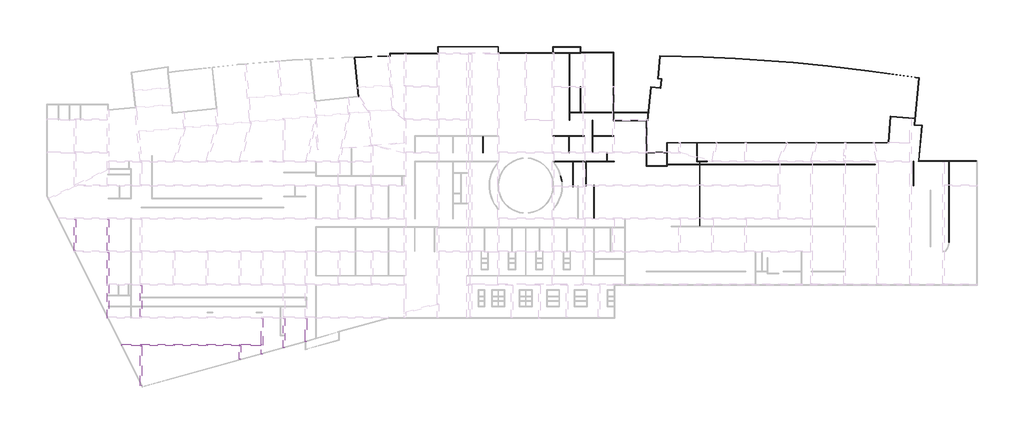
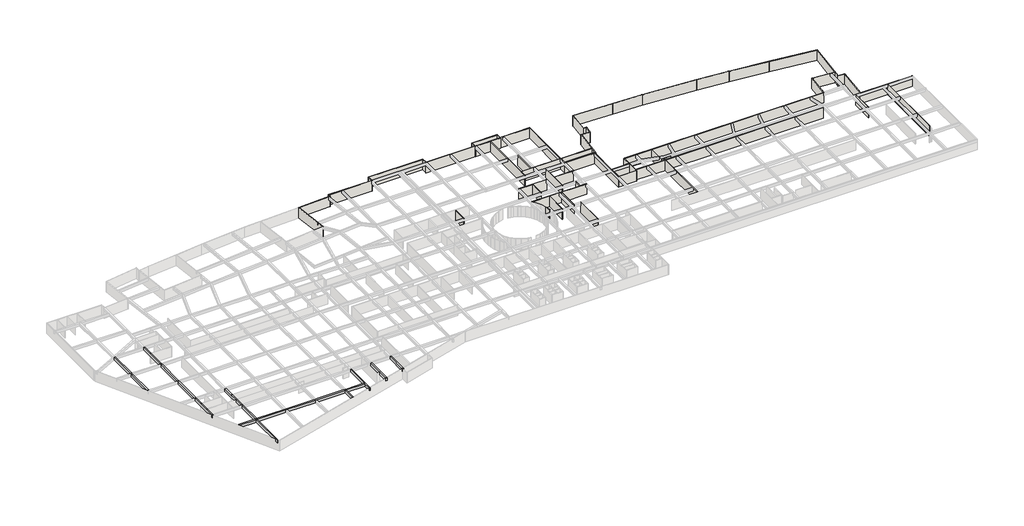
# One storey, part 4 of 8: 57 walls, 10 beams.
"""IFC4 building model written with IfcOpenShell, lengths in millimetres."""

from ifc_helpers import new_model, si_unit, frame, origin, origin_with_axes, place, context, project, spatial, polyline, outline, extrude, faceted_brep, element, save

model = new_model("IFC4")

# Units and contexts
model_context = context("Model", 3, world=origin())
ifc_project = project(units=[si_unit("LENGTHUNIT", "METRE", prefix="MILLI")], contexts=[model_context])

# Site, building, storey
site = spatial("IfcSite", under=ifc_project)
building = spatial("IfcBuilding", under=site)
storey = spatial("IfcBuildingStorey", under=building, Name="户型图", Elevation=0.0)

# Beams
placement = place(None, origin())
element("IfcBeam", 1, ObjectType="混凝土 - 矩形梁 : KL_beam", at=placement, inside=storey, context=model_context, shape_type="SweptSolid", body=[
    extrude(outline(polyline([(307553.8653555, -11261.3735096), (307153.8653555, -11261.3735096), (307153.8653555, -2661.3735096), (307553.8653555, -2661.3735096), (307553.8653555, -11261.3735096)])), frame((0.0, 0.0, 2500.0), z_axis=(0.0, 0.0, 1.0), x_axis=(1.0, 0.0, 0.0)), (0.0, 0.0, 1.0), 800.0),
    extrude(outline(polyline([(307153.8653555, 6215.0196927), (307401.078951, 6338.6264904), (307553.8653555, 6338.6264904), (307553.8653555, -2261.3735096), (307153.8653555, -2261.3735096), (307153.8653555, 6215.0196927)])), frame((0.0, 0.0, 2500.0), z_axis=(0.0, 0.0, 1.0), x_axis=(1.0, 0.0, 0.0)), (0.0, 0.0, 1.0), 800.0),
])
element("IfcBeam", 2, ObjectType="混凝土 - 矩形梁 : KL_beam", at=placement, inside=storey, context=model_context, shape_type="SweptSolid", body=[
    extrude(outline(polyline([(316153.8653576, 6338.6264904), (316553.8653576, 6338.6264904), (316553.8653576, -2261.3735096), (316153.8653576, -2261.3735096), (316153.8653576, 6338.6264904)])), frame((0.0, 0.0, 2500.0), z_axis=(0.0, 0.0, 1.0), x_axis=(1.0, 0.0, 0.0)), (0.0, 0.0, 1.0), 800.0),
    extrude(outline(polyline([(316553.8653576, -11261.3735096), (316153.8653576, -11261.3735096), (316153.8653576, -2661.3735096), (316553.8653576, -2661.3735096), (316553.8653576, -11261.3735096)])), frame((0.0, 0.0, 2500.0), z_axis=(0.0, 0.0, 1.0), x_axis=(1.0, 0.0, 0.0)), (0.0, 0.0, 1.0), 800.0),
])
element("IfcBeam", 3, ObjectType="混凝土 - 矩形梁 : KL_beam", at=placement, inside=storey, context=model_context, shape_type="Brep", body=[
    faceted_brep([(316153.8653576, -29635.5681734, 3300.0), (316553.8653576, -29635.5681734, 3300.0), (316553.8653576, -29235.5681734, 3300.0), (316553.8653576, -20661.3735124, 3300.0), (316553.8653576, -20261.3735124, 3300.0), (316553.8653576, -11661.3735096, 3300.0), (316153.8653576, -11661.3735096, 3300.0), (316153.8653576, -20261.3735124, 3300.0), (316153.8653576, -20661.3735124, 3300.0), (316153.8653576, -29635.5681734, 2500.0), (316153.8653576, -11661.3735096, 2500.0), (316153.8653576, -20261.3735124, 2500.0), (316153.8653576, -20661.3735124, 2500.0), (316553.8653576, -29635.5681734, 2500.0), (316553.8653576, -11661.3735096, 2500.0), (316553.8653576, -20261.3735124, 2500.0), (316553.8653576, -20661.3735124, 2500.0), (316553.8653576, -29235.5681734, 2500.0)], [[[0, 1, 2, 3, 4, 5, 6, 7, 8]], [[9, 0, 8, 7, 6, 10, 11, 12]], [[13, 9, 12, 11, 10, 14, 15, 16, 17]], [[1, 13, 17, 16, 15, 14, 5, 4, 3, 2]], [[6, 5, 14, 10]], [[1, 0, 9, 13]]]),
])
element("IfcBeam", 4, ObjectType="混凝土 - 矩形梁 : KL_beam", at=placement, inside=storey, context=model_context, shape_type="SweptSolid", body=[
    extrude(outline(polyline([(325153.8653576, -20661.3735124), (325553.8653576, -20661.3735124), (325553.8653576, -29235.5681734), (325153.8653576, -29235.5681734), (325153.8653576, -20661.3735124)])), frame((0.0, 0.0, 2500.0), z_axis=(0.0, 0.0, 1.0), x_axis=(1.0, 0.0, 0.0)), (0.0, 0.0, 1.0), 800.0),
    extrude(outline(polyline([(325153.8653576, -29635.5681734), (325553.8653576, -29635.5681734), (325553.8653576, -36750.8162358), (325153.8653576, -36750.8162358), (325153.8653576, -29635.5681734)])), frame((0.0, 0.0, 2500.0), z_axis=(0.0, 0.0, 1.0), x_axis=(1.0, 0.0, 0.0)), (0.0, 0.0, 1.0), 800.0),
])
element("IfcBeam", 5, ObjectType="混凝土 - 矩形梁 : KL_beam", at=placement, inside=storey, context=model_context, shape_type="SweptSolid", body=[
    extrude(outline(polyline([(325553.8653576, -48161.0948727), (325153.8653576, -48161.0948727), (325153.8653576, -37150.8162358), (325553.8653576, -37150.8162358), (325553.8653576, -48161.0948727)])), frame((0.0, 0.0, 2500.0), z_axis=(0.0, 0.0, 1.0), x_axis=(1.0, 0.0, 0.0)), (0.0, 0.0, 1.0), 800.0),
])
element("IfcBeam", 6, ObjectType="混凝土 - 矩形梁 : KL_beam", at=placement, inside=storey, context=model_context, shape_type="Brep", body=[
    faceted_brep([(320098.7260393, -36750.8162358, 3300.0), (320098.7260393, -36750.8162358, 2500.0), (320098.7260393, -37150.8162358, 2500.0), (320098.7260393, -37150.8162358, 3300.0), (325153.8653576, -37150.8162358, 3300.0), (325553.8653576, -37150.8162358, 3300.0), (334153.8653576, -37150.8162358, 3300.0), (334553.8653576, -37150.8162358, 3300.0), (343153.8653576, -37150.8162358, 3300.0), (343553.8653576, -37150.8162358, 3300.0), (352153.8653576, -37150.8162358, 3300.0), (352553.8653576, -37150.8162358, 3300.0), (358153.8653576, -37150.8162358, 3300.0), (358153.8653576, -36750.8162358, 3300.0), (352553.8653576, -36750.8162358, 3300.0), (352153.8653576, -36750.8162358, 3300.0), (343553.8653576, -36750.8162358, 3300.0), (343153.8653576, -36750.8162358, 3300.0), (334553.8653576, -36750.8162358, 3300.0), (334153.8653576, -36750.8162358, 3300.0), (325553.8653576, -36750.8162358, 3300.0), (325153.8653576, -36750.8162358, 3300.0), (325153.8653576, -37150.8162358, 2500.0), (325553.8653576, -37150.8162358, 2500.0), (334153.8653576, -37150.8162358, 2500.0), (334553.8653576, -37150.8162358, 2500.0), (343153.8653576, -37150.8162358, 2500.0), (343553.8653576, -37150.8162358, 2500.0), (352153.8653576, -37150.8162358, 2500.0), (352553.8653576, -37150.8162358, 2500.0), (358153.8653576, -37150.8162358, 2500.0), (325153.8653576, -36750.8162358, 2500.0), (325553.8653576, -36750.8162358, 2500.0), (334153.8653576, -36750.8162358, 2500.0), (334553.8653576, -36750.8162358, 2500.0), (343153.8653576, -36750.8162358, 2500.0), (343553.8653576, -36750.8162358, 2500.0), (352153.8653576, -36750.8162358, 2500.0), (352553.8653576, -36750.8162358, 2500.0), (358153.8653576, -36750.8162358, 2500.0)], [[[0, 1, 2, 3]], [[0, 3, 4, 5, 6, 7, 8, 9, 10, 11, 12, 13, 14, 15, 16, 17, 18, 19, 20, 21]], [[3, 2, 22, 23, 24, 25, 26, 27, 28, 29, 30, 12, 11, 10, 9, 8, 7, 6, 5, 4]], [[2, 1, 31, 32, 33, 34, 35, 36, 37, 38, 39, 30, 29, 28, 27, 26, 25, 24, 23, 22]], [[1, 0, 21, 20, 19, 18, 17, 16, 15, 14, 13, 39, 38, 37, 36, 35, 34, 33, 32, 31]], [[13, 12, 30, 39]]]),
])
element("IfcBeam", 7, ObjectType="混凝土 - 矩形梁 : KL_beam", at=placement, inside=storey, context=model_context, shape_type="SweptSolid", body=[
    extrude(outline(polyline([(352553.8653576, -40850.8162358), (352153.8653576, -40850.8162358), (352153.8653576, -37150.8162358), (352553.8653576, -37150.8162358), (352553.8653576, -40850.8162358)])), frame((0.0, 0.0, 2500.0), z_axis=(0.0, 0.0, 1.0), x_axis=(1.0, 0.0, 0.0)), (0.0, 0.0, 1.0), 800.0),
])
element("IfcBeam", 8, ObjectType="混凝土 - 矩形梁 : KL_beam", at=placement, inside=storey, context=model_context, shape_type="Brep", body=[
    faceted_brep([(358553.8653576, -39436.8004779, 3300.0), (358153.8653576, -39436.8004779, 3300.0), (358153.8653576, -39436.8004779, 2500.0), (358553.8653576, -39436.8004779, 2500.0), (358553.8653576, -29635.5681734, 3300.0), (358153.8653576, -29635.5681734, 3300.0), (358153.8653576, -36750.8162358, 3300.0), (358153.8653576, -37150.8162358, 3300.0), (358153.8653576, -29635.5681734, 2500.0), (358153.8653576, -36750.8162358, 2500.0), (358153.8653576, -37150.8162358, 2500.0), (358553.8653576, -29635.5681734, 2500.0)], [[[0, 1, 2, 3]], [[1, 0, 4, 5, 6, 7]], [[2, 1, 7, 6, 5, 8, 9, 10]], [[3, 2, 10, 9, 8, 11]], [[0, 3, 11, 4]], [[5, 4, 11, 8]]]),
])
element("IfcBeam", 9, ObjectType="混凝土 - 矩形梁 : KL_beam", at=placement, inside=storey, context=model_context, shape_type="SweptSolid", body=[
    extrude(outline(polyline([(364553.8653576, -37769.9671448), (364153.8653576, -37769.9671448), (364153.8653576, -29635.5681734), (364553.8653576, -29635.5681734), (364553.8653576, -37769.9671448)])), frame((0.0, 0.0, 2500.0), z_axis=(0.0, 0.0, 1.0), x_axis=(1.0, 0.0, 0.0)), (0.0, 0.0, 1.0), 800.0),
])
element("IfcBeam", 10, ObjectType="混凝土 - 矩形梁 : KL_beam", at=placement, inside=storey, context=model_context, shape_type="SweptSolid", body=[
    extrude(outline(polyline([(370553.8653576, -36103.6338116), (370153.8653576, -36103.6338116), (370153.8653576, -29635.5681734), (370553.8653576, -29635.5681734), (370553.8653576, -36103.6338116)])), frame((0.0, 0.0, 2500.0), z_axis=(0.0, 0.0, 1.0), x_axis=(1.0, 0.0, 0.0)), (0.0, 0.0, 1.0), 800.0),
])

# Walls
element("IfcWall", 11, ObjectType="所有墙体", at=placement, inside=storey, context=model_context, shape_type="Brep", body=[
    faceted_brep([(553458.7450641, 13292.21774, 0.0), (537684.2235741, 13292.21774, 0.0), (537563.7651936, 13292.21774, 0.0), (537563.7651936, 13292.21774, 3300.0), (537684.2235741, 13292.21774, 3300.0), (553458.7450641, 13292.21774, 3300.0), (553458.7450641, 13172.21774, 0.0), (553458.7450641, 13172.21774, 3300.0), (537553.266554, 13172.21774, 3300.0), (537553.266554, 13172.21774, 0.0)], [[[0, 1, 2, 3, 4, 5]], [[6, 7, 8, 9]], [[2, 1, 0, 6, 9]], [[5, 4, 3, 8, 7]], [[0, 5, 7, 6]], [[3, 2, 9, 8]]]),
])
element("IfcWall", 12, ObjectType="所有墙体", at=placement, inside=storey, context=model_context, shape_type="Brep", body=[
    faceted_brep([(537684.2235741, 13292.21774, 0.0), (538529.2876848, 22951.3447265, 0.0), (538529.2876848, 22951.3447265, 3300.0), (537684.2235741, 13292.21774, 3300.0), (537563.7651936, 13292.21774, 0.0), (537563.7651936, 13292.21774, 3300.0), (538399.3397888, 22842.8790687, 3300.0), (538409.7986189, 22962.4240435, 3300.0), (538409.7986189, 22962.4240435, 0.0), (538399.3397888, 22842.8790687, 0.0)], [[[0, 1, 2, 3]], [[4, 5, 6, 7, 8, 9]], [[1, 0, 4, 9, 8]], [[3, 2, 7, 6, 5]], [[0, 3, 5, 4]], [[2, 1, 8, 7]]]),
])
element("IfcWall", 13, ObjectType="所有墙体", at=placement, inside=storey, context=model_context, shape_type="Brep", body=[
    faceted_brep([(538409.7986189, 22962.4240435, 0.0), (536538.1394552, 23135.9688357, 0.0), (536418.6519996, 23147.0480034, 0.0), (536418.6519996, 23147.0480034, 3300.0), (536538.1394552, 23135.9688357, 3300.0), (538409.7986189, 22962.4240435, 3300.0), (538399.3397888, 22842.8790687, 0.0), (538399.3397888, 22842.8790687, 3300.0), (536407.572832, 23027.5605478, 3300.0), (536407.572832, 23027.5605478, 0.0)], [[[0, 1, 2, 3, 4, 5]], [[6, 7, 8, 9]], [[2, 1, 0, 6, 9]], [[5, 4, 3, 8, 7]], [[0, 5, 7, 6]], [[3, 2, 9, 8]]]),
])
element("IfcWall", 14, ObjectType="所有墙体", at=placement, inside=storey, context=model_context, shape_type="Brep", body=[
    faceted_brep([(536538.1394552, 23135.9688357, 0.0), (537732.2315967, 36014.1051945, 0.0), (537732.2315967, 36014.1051945, 3300.0), (536538.1394552, 23135.9688357, 3300.0), (536418.6519996, 23147.0480034, 0.0), (536418.6519996, 23147.0480034, 3300.0), (536566.2044403, 24738.382864, 3300.0), (536577.283608, 24857.8703196, 3300.0), (537602.1010394, 35910.3998237, 3300.0), (537613.1891402, 36029.9836226, 3300.0), (537613.1891402, 36029.9836226, 0.0), (537602.1010394, 35910.3998237, 0.0), (536577.283608, 24857.8703196, 0.0), (536566.2044403, 24738.382864, 0.0)], [[[0, 1, 2, 3]], [[4, 5, 6, 7, 8, 9, 10, 11, 12, 13]], [[1, 0, 4, 13, 12, 11, 10]], [[3, 2, 9, 8, 7, 6, 5]], [[0, 3, 5, 4]], [[2, 1, 10, 9]]]),
])
element("IfcWall", 15, ObjectType="所有墙体", at=placement, inside=storey, context=model_context, shape_type="SweptSolid", body=[
    extrude(outline(polyline([(524037.26481, 37840.8025861), (537613.1891402, 36029.9836226), (537602.1010394, 35910.3998237), (524021.9834406, 37721.7781046), (524037.26481, 37840.8025861)])), origin_with_axes(), (0.0, 0.0, 1.0), 3300.0),
])
element("IfcWall", 16, ObjectType="所有墙体", at=placement, inside=storey, context=model_context, shape_type="SweptSolid", body=[
    extrude(outline(polyline([(512770.3311829, 39231.1267428), (524037.26481, 37840.8025861), (524021.9834406, 37721.7781046), (512757.0555613, 39111.8547548), (512770.3311829, 39231.1267428)])), origin_with_axes(), (0.0, 0.0, 1.0), 3300.0),
])
element("IfcWall", 17, ObjectType="所有墙体", at=placement, inside=storey, context=model_context, shape_type="SweptSolid", body=[
    extrude(outline(polyline([(503394.9424706, 40161.5809347), (512770.3311829, 39231.1267428), (512757.0555613, 39111.8547548), (503384.5461664, 40042.0231907), (503394.9424706, 40161.5809347)])), origin_with_axes(), (0.0, 0.0, 1.0), 3300.0),
])
element("IfcWall", 18, ObjectType="所有墙体", at=placement, inside=storey, context=model_context, shape_type="SweptSolid", body=[
    extrude(outline(polyline([(487600.1090231, 41341.3659197), (503394.9424706, 40161.5809347), (503384.5461664, 40042.0231907), (487593.4285844, 41221.5306216), (487600.1090231, 41341.3659197)])), origin_with_axes(), (0.0, 0.0, 1.0), 3300.0),
])
element("IfcWall", 19, ObjectType="所有墙体", at=placement, inside=storey, context=model_context, shape_type="SweptSolid", body=[
    extrude(outline(polyline([(478777.792417, 41666.3723956), (487600.1090231, 41341.3659197), (487593.4285844, 41221.5306216), (478774.1034736, 41546.4268934), (478777.792417, 41666.3723956)])), origin_with_axes(), (0.0, 0.0, 1.0), 3300.0),
])
element("IfcWall", 20, ObjectType="所有墙体", at=placement, inside=storey, context=model_context, shape_type="Brep", body=[
    faceted_brep([(478777.792417, 41666.3723956, 0.0), (466951.5716276, 41958.1662767, 0.0), (466951.5716276, 41958.1662767, 3300.0), (478777.792417, 41666.3723956, 3300.0), (478774.1034736, 41546.4268934, 0.0), (478774.1034736, 41546.4268934, 3300.0), (467061.2925699, 41835.4225593, 3300.0), (466941.0937395, 41838.3882813, 3300.0), (466941.0937395, 41838.3882813, 0.0), (467061.2925699, 41835.4225593, 0.0)], [[[0, 1, 2, 3]], [[4, 5, 6, 7, 8, 9]], [[1, 0, 4, 9, 8]], [[3, 2, 7, 6, 5]], [[0, 3, 5, 4]], [[2, 1, 8, 7]]]),
])
element("IfcWall", 21, ObjectType="所有墙体", at=placement, inside=storey, context=model_context, shape_type="Brep", body=[
    faceted_brep([(466941.0937395, 41838.3882813, 0.0), (466401.1341207, 35665.8389465, 0.0), (466401.1341207, 35665.8389465, 3300.0), (466941.0937395, 41838.3882813, 3300.0), (467061.2925699, 41835.4225593, 0.0), (467061.2925699, 41835.4225593, 3300.0), (466531.1348575, 35774.9237362, 3300.0), (466520.6774844, 35655.3802573, 3300.0), (466520.6774844, 35655.3802573, 0.0), (466531.1348575, 35774.9237362, 0.0)], [[[0, 1, 2, 3]], [[4, 5, 6, 7, 8, 9]], [[1, 0, 4, 9, 8]], [[3, 2, 7, 6, 5]], [[0, 3, 5, 4]], [[2, 1, 8, 7]]]),
])
element("IfcWall", 22, ObjectType="所有墙体", at=placement, inside=storey, context=model_context, shape_type="Brep", body=[
    faceted_brep([(466520.6774844, 35655.3802573, 0.0), (467298.2016586, 35587.3557065, 0.0), (467417.7450224, 35576.8970174, 0.0), (467417.7450224, 35576.8970174, 3300.0), (467298.2016586, 35587.3557065, 3300.0), (466520.6774844, 35655.3802573, 3300.0), (466531.1348575, 35774.9237362, 0.0), (466531.1348575, 35774.9237362, 3300.0), (467428.2037115, 35696.4403811, 3300.0), (467428.2037115, 35696.4403811, 0.0)], [[[0, 1, 2, 3, 4, 5]], [[6, 7, 8, 9]], [[2, 1, 0, 6, 9]], [[5, 4, 3, 8, 7]], [[0, 5, 7, 6]], [[3, 2, 9, 8]]]),
])
element("IfcWall", 23, ObjectType="所有墙体", at=placement, inside=storey, context=model_context, shape_type="Brep", body=[
    faceted_brep([(467298.2016586, 35587.3557065, 0.0), (467095.1766515, 33266.769256, 0.0), (467084.7179624, 33147.2258923, 0.0), (467084.7179624, 33147.2258923, 3300.0), (467095.1766515, 33266.769256, 3300.0), (467298.2016586, 35587.3557065, 3300.0), (467417.7450224, 35576.8970174, 0.0), (467417.7450224, 35576.8970174, 3300.0), (467204.2613261, 33136.7672031, 3300.0), (467204.2613261, 33136.7672031, 0.0)], [[[0, 1, 2, 3, 4, 5]], [[6, 7, 8, 9]], [[2, 1, 0, 6, 9]], [[5, 4, 3, 8, 7]], [[0, 5, 7, 6]], [[3, 2, 9, 8]]]),
])
element("IfcWall", 24, ObjectType="所有墙体", at=placement, inside=storey, context=model_context, shape_type="Brep", body=[
    faceted_brep([(467095.1766515, 33266.769256, 0.0), (464505.7177262, 33493.3175566, 0.0), (464505.7177262, 33493.3175566, 3300.0), (467095.1766515, 33266.769256, 3300.0), (467084.7179624, 33147.2258923, 0.0), (467084.7179624, 33147.2258923, 3300.0), (464613.5078213, 33363.4287647, 3300.0), (464493.9573711, 33373.8880738, 3300.0), (464493.9573711, 33373.8880738, 0.0), (464613.5078213, 33363.4287647, 0.0)], [[[0, 1, 2, 3]], [[4, 5, 6, 7, 8, 9]], [[1, 0, 4, 9, 8]], [[3, 2, 7, 6, 5]], [[0, 3, 5, 4]], [[2, 1, 8, 7]]]),
])
element("IfcWall", 25, ObjectType="所有墙体", at=placement, inside=storey, context=model_context, shape_type="Brep", body=[
    faceted_brep([(464493.9573711, 33373.8880738, 0.0), (463826.7897593, 26598.6264677, 0.0), (463814.9732246, 26478.6264677, 0.0), (463600.3061777, 24298.6264562, 0.0), (463588.489643, 24178.6264562, 0.0), (463588.489643, 24178.6264562, 3300.0), (463600.3061777, 24298.6264562, 3300.0), (463814.9732246, 26478.6264677, 3300.0), (463826.7897593, 26598.6264677, 3300.0), (464493.9573711, 33373.8880738, 3300.0), (464613.5078213, 33363.4287647, 0.0), (464613.5078213, 33363.4287647, 3300.0), (463709.0700332, 24178.6264562, 3300.0), (463709.0700332, 24178.6264562, 0.0)], [[[0, 1, 2, 3, 4, 5, 6, 7, 8, 9]], [[10, 11, 12, 13]], [[4, 3, 2, 1, 0, 10, 13]], [[9, 8, 7, 6, 5, 12, 11]], [[0, 9, 11, 10]], [[5, 4, 13, 12]]]),
])
element("IfcWall", 26, ObjectType="所有墙体", at=placement, inside=storey, context=model_context, shape_type="Brep", body=[
    faceted_brep([(463600.3061777, 24298.6264562, 0.0), (454413.8653571, 24298.6264562, 0.0), (454293.8653571, 24298.6264562, 0.0), (454293.8653571, 24298.6264562, 3300.0), (454413.8653571, 24298.6264562, 3300.0), (463600.3061777, 24298.6264562, 3300.0), (463588.489643, 24178.6264562, 0.0), (463588.489643, 24178.6264562, 3300.0), (463413.8653576, 24178.6264562, 3300.0), (463293.8653576, 24178.6264562, 3300.0), (454293.8653571, 24178.6264562, 3300.0), (454293.8653571, 24178.6264562, 0.0), (463293.8653576, 24178.6264562, 0.0), (463413.8653576, 24178.6264562, 0.0)], [[[0, 1, 2, 3, 4, 5]], [[6, 7, 8, 9, 10, 11, 12, 13]], [[2, 1, 0, 6, 13, 12, 11]], [[5, 4, 3, 10, 9, 8, 7]], [[0, 5, 7, 6]], [[3, 2, 11, 10]]]),
])
element("IfcWall", 27, ObjectType="所有墙体", at=placement, inside=storey, context=model_context, shape_type="Brep", body=[
    faceted_brep([(454413.8653571, 24298.6264562, 0.0), (454413.8653571, 26478.6264677, 0.0), (454413.8653571, 26598.6264677, 0.0), (454413.8653571, 42898.6264606, 0.0), (454413.8653571, 42898.6264606, 3300.0), (454413.8653571, 26598.6264677, 3300.0), (454413.8653571, 26478.6264677, 3300.0), (454413.8653571, 24298.6264562, 3300.0), (454293.8653571, 24298.6264562, 0.0), (454293.8653571, 24298.6264562, 3300.0), (454293.8653571, 26478.6264677, 3300.0), (454293.8653571, 26598.6264677, 3300.0), (454293.8653571, 42778.6264606, 3300.0), (454293.8653571, 42898.6264606, 3300.0), (454293.8653571, 42898.6264606, 0.0), (454293.8653571, 42778.6264606, 0.0), (454293.8653571, 26598.6264677, 0.0), (454293.8653571, 26478.6264677, 0.0)], [[[0, 1, 2, 3, 4, 5, 6, 7]], [[8, 9, 10, 11, 12, 13, 14, 15, 16, 17]], [[3, 2, 1, 0, 8, 17, 16, 15, 14]], [[7, 6, 5, 4, 13, 12, 11, 10, 9]], [[0, 7, 9, 8]], [[4, 3, 14, 13]]]),
])
element("IfcWall", 28, ObjectType="所有墙体", at=placement, inside=storey, context=model_context, shape_type="Brep", body=[
    faceted_brep([(454293.8653571, 42898.6264606, 0.0), (445413.8653571, 42898.6264606, 0.0), (445293.8653571, 42898.6264606, 0.0), (445293.8653571, 42898.6264606, 3300.0), (445413.8653571, 42898.6264606, 3300.0), (454293.8653571, 42898.6264606, 3300.0), (454293.8653571, 42778.6264606, 0.0), (454293.8653571, 42778.6264606, 3300.0), (445293.8653571, 42778.6264606, 3300.0), (445293.8653571, 42778.6264606, 0.0)], [[[0, 1, 2, 3, 4, 5]], [[6, 7, 8, 9]], [[2, 1, 0, 6, 9]], [[5, 4, 3, 8, 7]], [[0, 5, 7, 6]], [[3, 2, 9, 8]]]),
])
element("IfcWall", 29, ObjectType="所有墙体", at=placement, inside=storey, context=model_context, shape_type="Brep", body=[
    faceted_brep([(445413.8653571, 42898.6264606, 0.0), (445413.8653571, 44395.5707464, 0.0), (445413.8653571, 44395.5707464, 3300.0), (445413.8653571, 42898.6264606, 3300.0), (445293.8653571, 42898.6264606, 0.0), (445293.8653571, 42898.6264606, 3300.0), (445293.8653571, 44275.5707464, 3300.0), (445293.8653571, 44395.5707464, 3300.0), (445293.8653571, 44395.5707464, 0.0), (445293.8653571, 44275.5707464, 0.0)], [[[0, 1, 2, 3]], [[4, 5, 6, 7, 8, 9]], [[1, 0, 4, 9, 8]], [[3, 2, 7, 6, 5]], [[0, 3, 5, 4]], [[2, 1, 8, 7]]]),
])
element("IfcWall", 30, ObjectType="所有墙体", at=placement, inside=storey, context=model_context, shape_type="Brep", body=[
    faceted_brep([(445293.8653571, 44395.5707464, 0.0), (437693.8653571, 44395.5707464, 0.0), (437693.8653571, 44395.5707464, 3300.0), (445293.8653571, 44395.5707464, 3300.0), (445293.8653571, 44275.5707464, 0.0), (445293.8653571, 44275.5707464, 3300.0), (437813.8653571, 44275.5707464, 3300.0), (437693.8653571, 44275.5707464, 3300.0), (437693.8653571, 44275.5707464, 0.0), (437813.8653571, 44275.5707464, 0.0)], [[[0, 1, 2, 3]], [[4, 5, 6, 7, 8, 9]], [[1, 0, 4, 9, 8]], [[3, 2, 7, 6, 5]], [[0, 3, 5, 4]], [[2, 1, 8, 7]]]),
])
element("IfcWall", 31, ObjectType="所有墙体", at=placement, inside=storey, context=model_context, shape_type="Brep", body=[
    faceted_brep([(437693.8653571, 44275.5707464, 0.0), (437693.8653571, 42795.5707464, 0.0), (437693.8653571, 42675.5707464, 0.0), (437693.8653571, 42675.5707464, 3300.0), (437693.8653571, 42795.5707464, 3300.0), (437693.8653571, 44275.5707464, 3300.0), (437813.8653571, 44275.5707464, 0.0), (437813.8653571, 44275.5707464, 3300.0), (437813.8653571, 42735.5707464, 3300.0), (437813.8653571, 42675.5707464, 3300.0), (437813.8653571, 42675.5707464, 0.0), (437813.8653571, 42735.5707464, 0.0)], [[[0, 1, 2, 3, 4, 5]], [[6, 7, 8, 9, 10, 11]], [[2, 1, 0, 6, 11, 10]], [[5, 4, 3, 9, 8, 7]], [[0, 5, 7, 6]], [[3, 2, 10, 9]]]),
])
element("IfcWall", 32, ObjectType="所有墙体", at=placement, inside=storey, context=model_context, shape_type="Brep", body=[
    faceted_brep([(437693.8653571, 42795.5707464, 0.0), (422913.8653571, 42795.5707464, 0.0), (422793.8653571, 42795.5707464, 0.0), (422793.8653571, 42795.5707464, 3300.0), (422913.8653571, 42795.5707464, 3300.0), (437693.8653571, 42795.5707464, 3300.0), (437693.8653571, 42675.5707464, 0.0), (437693.8653571, 42675.5707464, 3300.0), (422793.8653571, 42675.5707464, 3300.0), (422793.8653571, 42675.5707464, 0.0)], [[[0, 1, 2, 3, 4, 5]], [[6, 7, 8, 9]], [[2, 1, 0, 6, 9]], [[5, 4, 3, 8, 7]], [[0, 5, 7, 6]], [[3, 2, 9, 8]]]),
])
element("IfcWall", 33, ObjectType="所有墙体", at=placement, inside=storey, context=model_context, shape_type="Brep", body=[
    faceted_brep([(422913.8653571, 42795.5707464, 0.0), (422913.8653571, 44495.5707464, 0.0), (422913.8653571, 44495.5707464, 3300.0), (422913.8653571, 42795.5707464, 3300.0), (422793.8653571, 42795.5707464, 0.0), (422793.8653571, 42795.5707464, 3300.0), (422793.8653571, 44375.5707464, 3300.0), (422793.8653571, 44495.5707464, 3300.0), (422793.8653571, 44495.5707464, 0.0), (422793.8653571, 44375.5707464, 0.0)], [[[0, 1, 2, 3]], [[4, 5, 6, 7, 8, 9]], [[1, 0, 4, 9, 8]], [[3, 2, 7, 6, 5]], [[0, 3, 5, 4]], [[2, 1, 8, 7]]]),
])
element("IfcWall", 34, ObjectType="所有墙体", at=placement, inside=storey, context=model_context, shape_type="Brep", body=[
    faceted_brep([(422793.8653571, 44495.5707464, 0.0), (406293.8653571, 44495.5707464, 0.0), (406293.8653571, 44495.5707464, 3300.0), (422793.8653571, 44495.5707464, 3300.0), (422793.8653571, 44375.5707464, 0.0), (422793.8653571, 44375.5707464, 3300.0), (406413.8653571, 44375.5707464, 3300.0), (406293.8653571, 44375.5707464, 3300.0), (406293.8653571, 44375.5707464, 0.0), (406413.8653571, 44375.5707464, 0.0)], [[[0, 1, 2, 3]], [[4, 5, 6, 7, 8, 9]], [[1, 0, 4, 9, 8]], [[3, 2, 7, 6, 5]], [[0, 3, 5, 4]], [[2, 1, 8, 7]]]),
])
element("IfcWall", 35, ObjectType="所有墙体", at=placement, inside=storey, context=model_context, shape_type="Brep", body=[
    faceted_brep([(406293.8653571, 44375.5707464, 0.0), (406293.8653571, 42695.5707464, 0.0), (406293.8653571, 42575.5707464, 0.0), (406293.8653571, 42575.5707464, 3300.0), (406293.8653571, 42695.5707464, 3300.0), (406293.8653571, 44375.5707464, 3300.0), (406413.8653571, 44375.5707464, 0.0), (406413.8653571, 44375.5707464, 3300.0), (406413.8653571, 42575.5707464, 3300.0), (406413.8653571, 42575.5707464, 0.0)], [[[0, 1, 2, 3, 4, 5]], [[6, 7, 8, 9]], [[2, 1, 0, 6, 9]], [[5, 4, 3, 8, 7]], [[0, 5, 7, 6]], [[3, 2, 9, 8]]]),
])
element("IfcWall", 36, ObjectType="所有墙体", at=placement, inside=storey, context=model_context, shape_type="Brep", body=[
    faceted_brep([(406293.8653571, 42695.5707464, 0.0), (393193.8653571, 42695.5707464, 0.0), (393193.8653571, 42695.5707464, 3300.0), (406293.8653571, 42695.5707464, 3300.0), (406293.8653571, 42575.5707464, 0.0), (406293.8653571, 42575.5707464, 3300.0), (393313.8653571, 42575.5707464, 3300.0), (393193.8653571, 42575.5707464, 3300.0), (393193.8653571, 42575.5707464, 0.0), (393313.8653571, 42575.5707464, 0.0)], [[[0, 1, 2, 3]], [[4, 5, 6, 7, 8, 9]], [[1, 0, 4, 9, 8]], [[3, 2, 7, 6, 5]], [[0, 3, 5, 4]], [[2, 1, 8, 7]]]),
])
element("IfcWall", 37, ObjectType="所有墙体", at=placement, inside=storey, context=model_context, shape_type="Brep", body=[
    faceted_brep([(393193.8653571, 42575.5707464, 0.0), (393193.8653571, 41993.3912245, 0.0), (393193.8653571, 41873.3090682, 0.0), (393193.8653571, 41873.3090682, 3300.0), (393193.8653571, 41993.3912245, 3300.0), (393193.8653571, 42575.5707464, 3300.0), (393313.8653571, 42575.5707464, 0.0), (393313.8653571, 42575.5707464, 3300.0), (393313.8653571, 41877.7502684, 3300.0), (393313.8653571, 41877.7502684, 0.0)], [[[0, 1, 2, 3, 4, 5]], [[6, 7, 8, 9]], [[2, 1, 0, 6, 9]], [[5, 4, 3, 8, 7]], [[0, 5, 7, 6]], [[3, 2, 9, 8]]]),
])
element("IfcWall", 38, ObjectType="所有墙体", at=placement, inside=storey, context=model_context, shape_type="Brep", body=[
    faceted_brep([(393193.8653571, 41993.3912245, 0.0), (383558.0584634, 41636.7699948, 0.0), (383558.0584634, 41636.7699948, 3300.0), (393193.8653571, 41993.3912245, 3300.0), (393193.8653571, 41873.3090682, 0.0), (393193.8653571, 41873.3090682, 3300.0), (383626.8769002, 41519.2348089, 3300.0), (383562.9450973, 41516.8686928, 3300.0), (383562.9450973, 41516.8686928, 0.0), (383626.8769002, 41519.2348089, 0.0)], [[[0, 1, 2, 3]], [[4, 5, 6, 7, 8, 9]], [[1, 0, 4, 9, 8]], [[3, 2, 7, 6, 5]], [[0, 3, 5, 4]], [[2, 1, 8, 7]]]),
])
element("IfcWall", 39, ObjectType="所有墙体", at=placement, inside=storey, context=model_context, shape_type="Brep", body=[
    faceted_brep([(384756.3754813, 30760.3408142, 0.0), (383626.8769002, 41519.2348089, 0.0), (383626.8769002, 41519.2348089, 3300.0), (384756.3754813, 30760.3408142, 3300.0), (384637.0313479, 30747.8117356, 0.0), (384637.0313479, 30747.8117356, 3300.0), (384624.5022692, 30867.155869, 3300.0), (383506.7284721, 41514.3669361, 3300.0), (383506.7284721, 41514.3669361, 0.0), (384624.5022692, 30867.155869, 0.0), (383562.9450973, 41516.8686928, 0.0), (383562.9450972, 41516.8686928, 3300.0)], [[[0, 1, 2, 3]], [[4, 5, 6, 7, 8, 9]], [[1, 0, 4, 9, 8, 10]], [[3, 2, 11, 7, 6, 5]], [[2, 1, 10, 11]], [[10, 8, 7, 11]], [[0, 3, 5, 4]]]),
])
element("IfcWall", 40, ObjectType="所有墙体", at=placement, inside=storey, context=model_context, shape_type="Brep", body=[
    faceted_brep([(463293.8653576, 24178.6264562, 0.0), (463293.8653576, 11778.6265283, 0.0), (463293.8653576, 11778.6265283, 3300.0), (463293.8653576, 24178.6264562, 3300.0), (463413.8653576, 24178.6264562, 0.0), (463413.8653576, 24178.6264562, 3300.0), (463413.8653576, 15598.6264904, 3300.0), (463413.8653576, 15478.6264904, 3300.0), (463413.8653576, 11898.6265283, 3300.0), (463413.8653576, 11778.6265283, 3300.0), (463413.8653576, 11778.6265283, 0.0), (463413.8653576, 11898.6265283, 0.0), (463413.8653576, 15478.6264904, 0.0), (463413.8653576, 15598.6264904, 0.0)], [[[0, 1, 2, 3]], [[4, 5, 6, 7, 8, 9, 10, 11, 12, 13]], [[1, 0, 4, 13, 12, 11, 10]], [[3, 2, 9, 8, 7, 6, 5]], [[0, 3, 5, 4]], [[2, 1, 10, 9]]]),
])
element("IfcWall", 41, ObjectType="所有墙体", at=placement, inside=storey, context=model_context, shape_type="SweptSolid", body=[
    extrude(outline(polyline([(468793.8653361, 15478.6264904), (463413.8653576, 15478.6264904), (463413.8653576, 15598.6264904), (468793.8653361, 15598.6264904), (468793.8653361, 15478.6264904)])), origin_with_axes(), (0.0, 0.0, 1.0), 3300.0),
])
element("IfcWall", 42, ObjectType="所有墙体", at=placement, inside=storey, context=model_context, shape_type="Brep", body=[
    faceted_brep([(468913.8653361, 11778.6265283, 0.0), (468913.8653361, 18178.6264904, 0.0), (468913.8653361, 18298.6264904, 0.0), (468913.8653361, 18298.6264904, 3300.0), (468913.8653361, 18178.6264904, 3300.0), (468913.8653361, 11778.6265283, 3300.0), (468793.8653361, 11778.6265283, 0.0), (468793.8653361, 11778.6265283, 3300.0), (468793.8653361, 11898.6265283, 3300.0), (468793.8653361, 15478.6264904, 3300.0), (468793.8653361, 15598.6264904, 3300.0), (468793.8653361, 18298.6264904, 3300.0), (468793.8653361, 18298.6264904, 0.0), (468793.8653361, 15598.6264904, 0.0), (468793.8653361, 15478.6264904, 0.0), (468793.8653361, 11898.6265283, 0.0)], [[[0, 1, 2, 3, 4, 5]], [[6, 7, 8, 9, 10, 11, 12, 13, 14, 15]], [[2, 1, 0, 6, 15, 14, 13, 12]], [[5, 4, 3, 11, 10, 9, 8, 7]], [[3, 2, 12, 11]], [[0, 5, 7, 6]]]),
])
element("IfcWall", 43, ObjectType="所有墙体", at=placement, inside=storey, context=model_context, shape_type="Brep", body=[
    faceted_brep([(468913.8653361, 18178.6264904, 0.0), (477093.8653576, 18178.6264904, 0.0), (477213.8653576, 18178.6264904, 0.0), (529386.6252053, 18178.6264904, 0.0), (529386.6252053, 18178.6264904, 3300.0), (477213.8653576, 18178.6264904, 3300.0), (477093.8653576, 18178.6264904, 3300.0), (468913.8653361, 18178.6264904, 3300.0), (468913.8653361, 18298.6264904, 0.0), (468913.8653361, 18298.6264904, 3300.0), (529276.7559158, 18298.6264904, 3300.0), (529397.2229767, 18298.6264904, 3300.0), (529397.2229767, 18298.6264904, 0.0), (529276.7559158, 18298.6264904, 0.0)], [[[0, 1, 2, 3, 4, 5, 6, 7]], [[8, 9, 10, 11, 12, 13]], [[3, 2, 1, 0, 8, 13, 12]], [[7, 6, 5, 4, 11, 10, 9]], [[0, 7, 9, 8]], [[4, 3, 12, 11]]]),
])
element("IfcWall", 44, ObjectType="所有墙体", at=placement, inside=storey, context=model_context, shape_type="Brep", body=[
    faceted_brep([(529397.2229767, 18298.6264904, 0.0), (530019.5574453, 25345.4039043, 0.0), (530030.1142291, 25464.9397966, 0.0), (530030.1142291, 25464.9397966, 3300.0), (530019.5574453, 25345.4039043, 3300.0), (529397.2229767, 18298.6264904, 3300.0), (529276.7559158, 18298.6264904, 0.0), (529276.7559158, 18298.6264904, 3300.0), (529910.6256316, 25476.0190701, 3300.0), (529910.6256316, 25476.0190701, 0.0)], [[[0, 1, 2, 3, 4, 5]], [[6, 7, 8, 9]], [[2, 1, 0, 6, 9]], [[5, 4, 3, 8, 7]], [[0, 5, 7, 6]], [[3, 2, 9, 8]]]),
])
element("IfcWall", 45, ObjectType="所有墙体", at=placement, inside=storey, context=model_context, shape_type="SweptSolid", body=[
    extrude(outline(polyline([(536566.2044403, 24738.382864), (530019.5574453, 25345.4039043), (530030.1142291, 25464.9397966), (536577.283608, 24857.8703196), (536566.2044403, 24738.382864)])), origin_with_axes(), (0.0, 0.0, 1.0), 3300.0),
])
element("IfcWall", 46, ObjectType="所有墙体", at=placement, inside=storey, context=model_context, shape_type="SweptSolid", body=[
    extrude(outline(polyline([(463413.8653576, 11898.6265283), (468793.8653361, 11898.6265283), (468793.8653361, 11778.6265283), (463413.8653576, 11778.6265283), (463413.8653576, 11898.6265283)])), origin_with_axes(), (0.0, 0.0, 1.0), 3300.0),
])
element("IfcWall", 47, ObjectType="所有墙体", at=placement, inside=storey, context=model_context, shape_type="Brep", body=[
    faceted_brep([(469204.0947142, 12228.624256, 0.0), (477798.5776142, 12228.624256, 0.0), (477918.5776142, 12228.624256, 0.0), (525704.0947142, 12228.624256, 0.0), (525704.0947142, 12228.624256, 3300.0), (477918.5776142, 12228.624256, 3300.0), (477798.5776142, 12228.624256, 3300.0), (469204.0947142, 12228.624256, 3300.0), (469204.0947142, 12348.624256, 0.0), (469204.0947142, 12348.624256, 3300.0), (477798.5776142, 12348.624256, 3300.0), (477918.5776142, 12348.624256, 3300.0), (525704.0947142, 12348.624256, 3300.0), (525704.0947142, 12348.624256, 0.0), (477918.5776142, 12348.624256, 0.0), (477798.5776142, 12348.624256, 0.0)], [[[0, 1, 2, 3, 4, 5, 6, 7]], [[8, 9, 10, 11, 12, 13, 14, 15]], [[3, 2, 1, 0, 8, 15, 14, 13]], [[4, 3, 13, 12]], [[7, 6, 5, 4, 12, 11, 10, 9]], [[0, 7, 9, 8]]]),
])
element("IfcWall", 48, ObjectType="所有墙体", at=placement, inside=storey, context=model_context, shape_type="Brep", body=[
    faceted_brep([(477093.8653576, 18178.6264904, 0.0), (477093.8653576, 13078.6264904, 0.0), (477093.8653576, 13078.6264904, 3300.0), (477093.8653576, 18178.6264904, 3300.0), (477213.8653576, 18178.6264904, 0.0), (477213.8653576, 18178.6264904, 3300.0), (477213.8653576, 13198.6264904, 3300.0), (477213.8653576, 13078.6264904, 3300.0), (477213.8653576, 13078.6264904, 0.0), (477213.8653576, 13198.6264904, 0.0)], [[[0, 1, 2, 3]], [[4, 5, 6, 7, 8, 9]], [[1, 0, 4, 9, 8]], [[3, 2, 7, 6, 5]], [[0, 3, 5, 4]], [[2, 1, 8, 7]]]),
])
element("IfcWall", 49, ObjectType="所有墙体", at=placement, inside=storey, context=model_context, shape_type="Brep", body=[
    faceted_brep([(477213.8653576, 13078.6264904, 0.0), (477798.5776142, 13078.6264904, 0.0), (477918.5776142, 13078.6264904, 0.0), (479953.8653576, 13078.6264904, 0.0), (479953.8653576, 13078.6264904, 3300.0), (477918.5776142, 13078.6264904, 3300.0), (477798.5776142, 13078.6264904, 3300.0), (477213.8653576, 13078.6264904, 3300.0), (477213.8653576, 13198.6264904, 0.0), (477213.8653576, 13198.6264904, 3300.0), (479953.8653576, 13198.6264904, 3300.0), (479953.8653576, 13198.6264904, 0.0)], [[[0, 1, 2, 3, 4, 5, 6, 7]], [[8, 9, 10, 11]], [[3, 2, 1, 0, 8, 11]], [[4, 3, 11, 10]], [[7, 6, 5, 4, 10, 9]], [[0, 7, 9, 8]]]),
])
element("IfcWall", 50, ObjectType="所有墙体", at=placement, inside=storey, context=model_context, shape_type="SweptSolid", body=[
    extrude(outline(polyline([(477798.5776142, 13078.6264904), (477918.5776142, 13078.6264904), (477918.5776142, 12348.624256), (477798.5776142, 12348.624256), (477798.5776142, 13078.6264904)])), origin_with_axes(), (0.0, 0.0, 1.0), 3300.0),
    extrude(outline(polyline([(477918.5776142, -4600.6191139), (477798.5776142, -4600.6191139), (477798.5776142, 12228.624256), (477918.5776142, 12228.624256), (477918.5776142, -4600.6191139)])), origin_with_axes(), (0.0, 0.0, 1.0), 3300.0),
])
element("IfcWall", 51, ObjectType="所有墙体", at=placement, inside=storey, context=model_context, shape_type="SweptSolid", body=[
    extrude(outline(polyline([(545793.8653576, -9056.1241898), (545793.8653576, 13138.6264904), (545913.8653576, 13138.6264904), (545913.8653576, -9066.6228294), (545793.8653576, -9056.1241898)])), origin_with_axes(), (0.0, 0.0, 1.0), 3300.0),
])
element("IfcWall", 52, ObjectType="所有墙体", at=placement, inside=storey, context=model_context, shape_type="SweptSolid", body=[
    extrude(outline(polyline([(440147.6903543, 7621.2941439), (439792.7443416, 9224.5035292), (439908.6998925, 9255.8962932), (440267.6903543, 7634.4190627), (440147.6903543, 7621.2941439)])), origin_with_axes(), (0.0, 0.0, 1.0), 3300.0),
])
element("IfcWall", 53, ObjectType="所有墙体", at=placement, inside=storey, context=model_context, shape_type="Brep", body=[
    faceted_brep([(437965.8355251, 13078.6264904, 0.0), (443193.8653576, 13078.6264904, 0.0), (443313.8653576, 13078.6264904, 0.0), (446793.8653576, 13078.6264904, 0.0), (446913.8653576, 13078.6264904, 0.0), (454453.8653576, 13078.6264904, 0.0), (454453.8653576, 13078.6264904, 3300.0), (446913.8653576, 13078.6264904, 3300.0), (446793.8653576, 13078.6264904, 3300.0), (443313.8653576, 13078.6264904, 3300.0), (443193.8653576, 13078.6264904, 3300.0), (437965.8355251, 13078.6264904, 3300.0), (437886.0167787, 13198.6264904, 0.0), (437886.0167787, 13198.6264904, 3300.0), (452493.8653576, 13198.6264904, 3300.0), (452613.8653576, 13198.6264904, 3300.0), (454453.8653576, 13198.6264904, 3300.0), (454453.8653576, 13198.6264904, 0.0), (452613.8653576, 13198.6264904, 0.0), (452493.8653576, 13198.6264904, 0.0)], [[[0, 1, 2, 3, 4, 5, 6, 7, 8, 9, 10, 11]], [[12, 13, 14, 15, 16, 17, 18, 19]], [[5, 4, 3, 2, 1, 0, 12, 19, 18, 17]], [[6, 5, 17, 16]], [[11, 10, 9, 8, 7, 6, 16, 15, 14, 13]], [[0, 11, 13, 12]]]),
])
element("IfcWall", 54, ObjectType="所有墙体", at=placement, inside=storey, context=model_context, shape_type="SweptSolid", body=[
    extrude(outline(polyline([(452613.8653576, 15438.6264904), (452613.8653576, 13198.6264904), (452493.8653576, 13198.6264904), (452493.8653576, 15438.6264904), (452613.8653576, 15438.6264904)])), origin_with_axes(), (0.0, 0.0, 1.0), 3300.0),
])
element("IfcWall", 55, ObjectType="所有墙体", at=placement, inside=storey, context=model_context, shape_type="SweptSolid", body=[
    extrude(outline(polyline([(446793.8653576, 6438.6264904), (446793.8653576, 13078.6264904), (446913.8653576, 13078.6264904), (446913.8653576, 6438.6264904), (446793.8653576, 6438.6264904)])), origin_with_axes(), (0.0, 0.0, 1.0), 3300.0),
])
element("IfcWall", 56, ObjectType="所有墙体", at=placement, inside=storey, context=model_context, shape_type="SweptSolid", body=[
    extrude(outline(polyline([(443193.8653576, 6288.6264674), (443193.8653576, 13078.6264904), (443313.8653576, 13078.6264904), (443313.8653576, 6288.6264674), (443193.8653576, 6288.6264674)])), origin_with_axes(), (0.0, 0.0, 1.0), 3300.0),
])
element("IfcWall", 57, ObjectType="所有墙体", at=placement, inside=storey, context=model_context, shape_type="SweptSolid", body=[
    extrude(outline(polyline([(448893.8653567, -2361.3735096), (448893.8653567, 6638.6264904), (449013.8653567, 6638.6264904), (449013.8653567, -2361.3735096), (448893.8653567, -2361.3735096)])), origin_with_axes(), (0.0, 0.0, 1.0), 3300.0),
])
element("IfcWall", 58, ObjectType="所有墙体", at=placement, inside=storey, context=model_context, shape_type="SweptSolid", body=[
    extrude(outline(polyline([(418593.8653576, 15438.6264906), (418593.8653576, 19978.6264904), (418713.8653576, 19978.6264904), (418713.8653576, 15438.6264906), (418593.8653576, 15438.6264906)])), origin_with_axes(), (0.0, 0.0, 1.0), 3300.0),
])
element("IfcWall", 59, ObjectType="所有墙体", at=placement, inside=storey, context=model_context, shape_type="Brep", body=[
    faceted_brep([(437813.8653571, 42615.5707464, 0.0), (442293.8653573, 42615.5707464, 0.0), (442413.8653573, 42615.5707464, 0.0), (445413.8653571, 42615.5707464, 0.0), (445413.8653571, 42615.5707464, 3300.0), (442413.8653573, 42615.5707464, 3300.0), (442293.8653573, 42615.5707464, 3300.0), (437813.8653571, 42615.5707464, 3300.0), (437813.8653571, 42735.5707464, 0.0), (437813.8653571, 42735.5707464, 3300.0), (445413.8653571, 42735.5707464, 3300.0), (445413.8653571, 42735.5707464, 0.0), (437813.8653571, 42675.5707464, 0.0), (437813.8653571, 42675.5707464, 3300.0)], [[[0, 1, 2, 3, 4, 5, 6, 7]], [[8, 9, 10, 11]], [[3, 2, 1, 0, 12, 8, 11]], [[4, 3, 11, 10]], [[7, 6, 5, 4, 10, 9, 13]], [[0, 7, 13, 9, 8, 12]]]),
])
element("IfcWall", 60, ObjectType="所有墙体", at=placement, inside=storey, context=model_context, shape_type="Brep", body=[
    faceted_brep([(442293.8653573, 42615.5707464, 0.0), (442293.8653573, 24438.6264904, 0.0), (442293.8653573, 24438.6264904, 3300.0), (442293.8653573, 42615.5707464, 3300.0), (442413.8653573, 42615.5707464, 0.0), (442413.8653573, 42615.5707464, 3300.0), (442413.8653573, 26598.6264677, 3300.0), (442413.8653573, 26478.6264677, 3300.0), (442413.8653573, 24438.6264904, 3300.0), (442413.8653573, 24438.6264904, 0.0), (442413.8653573, 26478.6264677, 0.0), (442413.8653573, 26598.6264677, 0.0)], [[[0, 1, 2, 3]], [[4, 5, 6, 7, 8, 9, 10, 11]], [[1, 0, 4, 11, 10, 9]], [[2, 1, 9, 8]], [[3, 2, 8, 7, 6, 5]], [[0, 3, 5, 4]]]),
])
element("IfcWall", 61, ObjectType="所有墙体", at=placement, inside=storey, context=model_context, shape_type="Brep", body=[
    faceted_brep([(463814.9732246, 26478.6264677, 0.0), (463814.9732246, 26478.6264677, 3300.0), (454413.8653571, 26478.6264677, 3300.0), (454413.8653571, 26478.6264677, 0.0), (463826.7897593, 26598.6264677, 3300.0), (463826.7897593, 26598.6264677, 0.0), (454413.8653571, 26598.6264677, 0.0), (454413.8653571, 26598.6264677, 3300.0)], [[[0, 1, 2, 3]], [[4, 5, 6, 7]], [[5, 0, 3, 6]], [[1, 4, 7, 2]], [[1, 0, 5, 4]], [[3, 2, 7, 6]]]),
    faceted_brep([(442413.8653573, 26478.6264677, 3300.0), (442413.8653573, 26478.6264677, 0.0), (454293.8653571, 26478.6264677, 0.0), (454293.8653571, 26478.6264677, 3300.0), (442413.8653573, 26598.6264677, 0.0), (442413.8653573, 26598.6264677, 3300.0), (445293.8653576, 26598.6264677, 3300.0), (445413.8653576, 26598.6264677, 3300.0), (454293.8653571, 26598.6264677, 3300.0), (454293.8653571, 26598.6264677, 0.0), (445413.8653576, 26598.6264677, 0.0), (445293.8653576, 26598.6264677, 0.0)], [[[0, 1, 2, 3]], [[4, 5, 6, 7, 8, 9, 10, 11]], [[1, 4, 11, 10, 9, 2]], [[5, 0, 3, 8, 7, 6]], [[1, 0, 5, 4]], [[3, 2, 9, 8]]]),
])
element("IfcWall", 62, ObjectType="所有墙体", at=placement, inside=storey, context=model_context, shape_type="SweptSolid", body=[
    extrude(outline(polyline([(445413.8653576, 33488.6264755), (445413.8653576, 26598.6264677), (445293.8653576, 26598.6264677), (445293.8653576, 33488.6264755), (445413.8653576, 33488.6264755)])), origin_with_axes(), (0.0, 0.0, 1.0), 3300.0),
])
element("IfcWall", 63, ObjectType="所有墙体", at=placement, inside=storey, context=model_context, shape_type="Brep", body=[
    faceted_brep([(437853.8653576, 19978.6264904, 0.0), (442043.8653576, 19978.6264904, 0.0), (442163.8653576, 19978.6264904, 0.0), (446353.8653576, 19978.6264904, 0.0), (446353.8653576, 19978.6264904, 3300.0), (442163.8653576, 19978.6264904, 3300.0), (442043.8653576, 19978.6264904, 3300.0), (437853.8653576, 19978.6264904, 3300.0), (437853.8653576, 20098.6264904, 0.0), (437853.8653576, 20098.6264904, 3300.0), (446353.8653576, 20098.6264904, 3300.0), (446353.8653576, 20098.6264904, 0.0)], [[[0, 1, 2, 3, 4, 5, 6, 7]], [[8, 9, 10, 11]], [[3, 2, 1, 0, 8, 11]], [[4, 3, 11, 10]], [[7, 6, 5, 4, 10, 9]], [[0, 7, 9, 8]]]),
])
element("IfcWall", 64, ObjectType="所有墙体", at=placement, inside=storey, context=model_context, shape_type="SweptSolid", body=[
    extrude(outline(polyline([(442043.8653576, 15538.6264904), (442043.8653576, 19978.6264904), (442163.8653576, 19978.6264904), (442163.8653576, 15538.6264904), (442043.8653576, 15538.6264904)])), origin_with_axes(), (0.0, 0.0, 1.0), 3300.0),
])
element("IfcWall", 65, ObjectType="所有墙体", at=placement, inside=storey, context=model_context, shape_type="Brep", body=[
    faceted_brep([(448613.8653576, 15538.6264904, 0.0), (448613.8653576, 19978.6264904, 0.0), (448613.8653576, 20098.6264904, 0.0), (448613.8653576, 24338.6264594, 0.0), (448613.8653576, 24338.6264594, 3300.0), (448613.8653576, 20098.6264904, 3300.0), (448613.8653576, 19978.6264904, 3300.0), (448613.8653576, 15538.6264904, 3300.0), (448493.8653576, 15538.6264904, 0.0), (448493.8653576, 15538.6264904, 3300.0), (448493.8653576, 24338.6264594, 3300.0), (448493.8653576, 24338.6264594, 0.0)], [[[0, 1, 2, 3, 4, 5, 6, 7]], [[8, 9, 10, 11]], [[3, 2, 1, 0, 8, 11]], [[4, 3, 11, 10]], [[7, 6, 5, 4, 10, 9]], [[0, 7, 9, 8]]]),
])
element("IfcWall", 66, ObjectType="所有墙体", at=placement, inside=storey, context=model_context, shape_type="SweptSolid", body=[
    extrude(outline(polyline([(454353.8653576, 19978.6264904), (448613.8653576, 19978.6264904), (448613.8653576, 20098.6264904), (454353.8653576, 20098.6264904), (454353.8653576, 19978.6264904)])), origin_with_axes(), (0.0, 0.0, 1.0), 3300.0),
])
element("IfcWall", 67, ObjectType="所有墙体", at=placement, inside=storey, context=model_context, shape_type="SweptSolid", body=[
    extrude(outline(polyline([(536213.8653576, 13138.6264904), (536213.8653576, 6538.6264904), (536093.8653576, 6538.6264904), (536093.8653576, 13138.6264904), (536213.8653576, 13138.6264904)])), origin_with_axes(), (0.0, 0.0, 1.0), 3300.0),
])

save(model, "model.ifc")

# Revit data of these elements
# Type "混凝土 - 矩形梁 : KL_beam"
#   Length [instance default] = 1524 mm
#   b = 400 mm
#   h = 800 mm
#   Structural Material [instance default] = 混凝土 - 现场浇注混凝土
#   Assembly Code = ""
# Type "所有墙体"
#   Layers, outside or top first: 120 mm "默认" (function 1)
# Elements 1, 2, 3, 4, 5, 6, 7, 8, 9, 10 (IfcBeam, "混凝土 - 矩形梁 : KL_beam")
#   Comments = ""
#   Structural Material = none
#   Phase Created = 新构造
# Elements 11, 12, 13, 14, 15, 16, 17, 18, 19, 20, 21, 22, 23, 24, 25, 26, 27, 28, 29, 30, 31, 32, 33, 34, 35, 36, 37, 38, 39, 40, 41, 42, 43, 44, 45, 46, 47, 48, 49, 50, 51, 52, 53, 54, 55, 56, 57, 58, 59, 60, 61, 62, 63, 64, 65, 66, 67 (IfcWall, "所有墙体")
#   Top Offset = 0 mm
#   Base Offset = 0 mm
#   wall height = 3300 mm
#   Phase Created = 新构造
#   Base Constraint = 户型图
#   Top Constraint = 层高
#   Materials on its faces: "默认"
# Materials
#   "混凝土 - 现场浇注混凝土": class "混凝土", colour RGB 192 192 192, transparency 0
#   "默认": class "其他", colour RGB 192 192 192, transparency 0, Cost = 0
